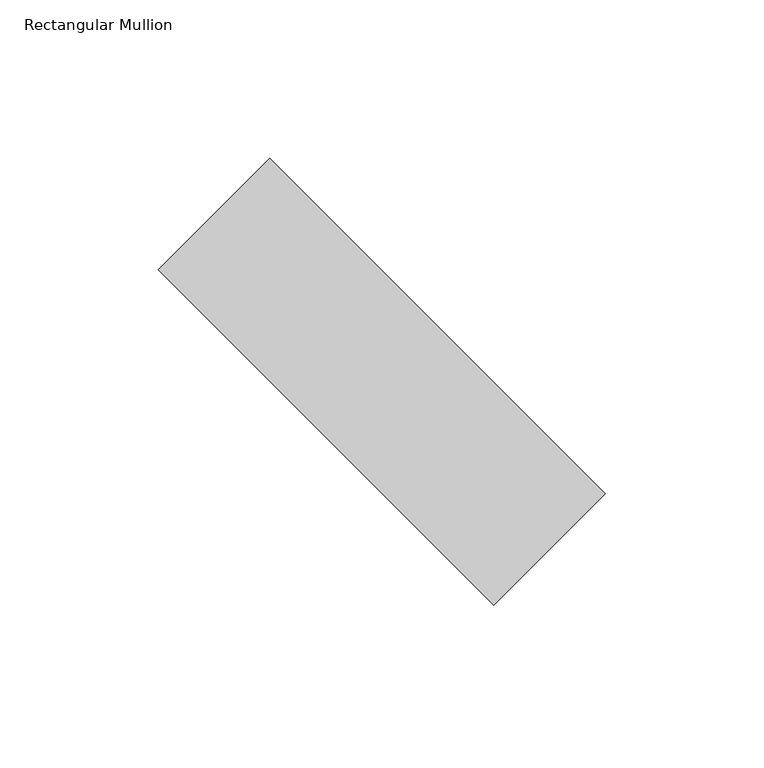
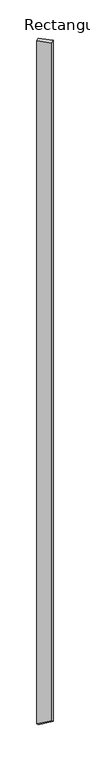
"""IFC4 building model written with IfcOpenShell, lengths in millimetres: member geometry, Rectangular Mullion : tilted mullions."""

from ifc_helpers import new_model, si_unit, origin, place, context, project, spatial, faceted_brep, source, transform, mapped, element, save


def rectangular_mullion_0aeb11d4(model_context):
    return source(origin(), model_context, "Body", "Brep", [
        faceted_brep([(-35.3553391, 70.7106781, 0.0), (-70.7106781, 35.3553391, 0.0), (35.3553391, -70.7106781, 0.0), (70.7106781, -35.3553391, 0.0), (-35.3553391, 70.7106781, -8054.6408326), (-70.7106781, 35.3553391, -8009.6306708), (35.3553391, -70.7106781, -7944.3101686), (70.7106781, -35.3553391, -7989.3203304)], [[[0, 1, 2, 3]], [[1, 0, 4, 5]], [[2, 1, 5, 6]], [[3, 2, 6, 7]], [[0, 3, 7, 4]], [[4, 7, 6, 5]]]),
    ])


if __name__ == "__main__":
    model = new_model("IFC4")
    model_context = context("Model", 3, world=origin())
    ifc_project = project(units=[si_unit("LENGTHUNIT", "METRE", prefix="MILLI")], contexts=[model_context])
    site = spatial("IfcSite", under=ifc_project)
    building = spatial("IfcBuilding", under=site)
    placement = place(None, origin())
    rectangular_mullion_shape = rectangular_mullion_0aeb11d4(model_context)
    element("IfcMember", 1, ObjectType="Rectangular Mullion : tilted mullions", at=placement, inside=building, context=model_context, shape_type="MappedRepresentation", body=[
        mapped(rectangular_mullion_shape, transform((0.0, 0.0, 0.0), x_axis=(1.0, 0.0, 0.0), y_axis=(0.0, 1.0, 0.0), z_axis=(0.0, 0.0, 1.0))),
    ])
    save(model, "model.ifc")

# Revit data of these elements
# Type "Rectangular Mullion : tilted mullions"
#   built-in parameter 1007304 = 0.492126 (stored number, unit not read)
#   built-in parameter 1007301 = 0.082021 (stored number, unit not read)
#   built-in parameter 1007300 = 0.082021 (stored number, unit not read)
# Element 1 (IfcMember, "Rectangular Mullion : tilted mullions")
#   Materials on its faces: "Aluminum"
# Materials
#   "Aluminum": class "Metal", colour RGB 244 244 244, transparency 0, Description = "Aluminum 6061", Cost = 0
